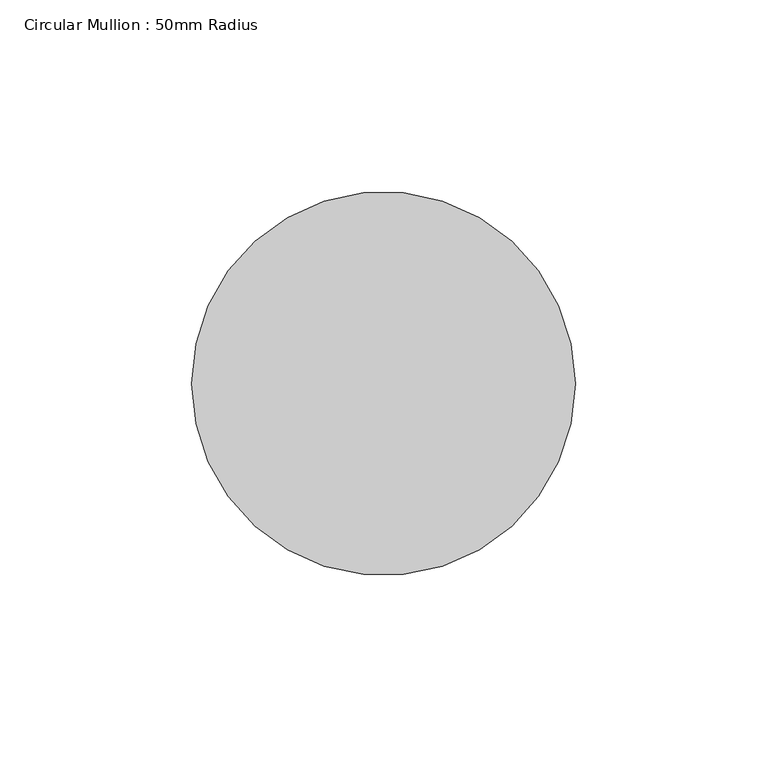
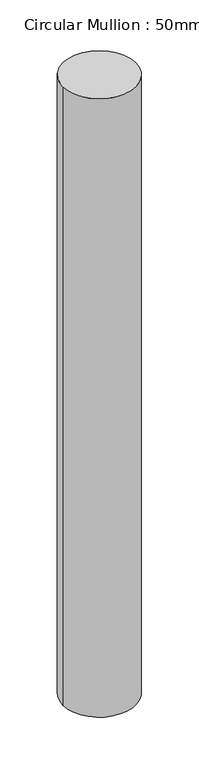
"""IFC4 building model written with IfcOpenShell, lengths in millimetres: member geometry, Circular Mullion : 50mm Radius."""

from ifc_helpers import new_model, si_unit, point, frame, origin, origin_2d, place, context, project, spatial, circle_curve, trimmed, segment, composite_curve, outline, extrude, source, transform, mapped, element, save


def circular_mullion_50mm_radius_ff912db3(model_context):
    return source(origin(), model_context, "Body", "SweptSolid", [
        extrude(outline(composite_curve([segment(trimmed(circle_curve(origin_2d(), 50.0), [point((50.0, 0.0))], [point((-50.0, 0.0))], False, "CARTESIAN"), True, "CONTINUOUS"), segment(trimmed(circle_curve(origin_2d(), 50.0), [point((-50.0, 0.0))], [point((50.0, 0.0))], False, "CARTESIAN"), True, "CONTINUOUS")], self_intersect=False)), frame((0.0, 0.0, -899.0118356), z_axis=(0.0, 0.0, 1.0), x_axis=(1.0, 0.0, 0.0)), (0.0, 0.0, 1.0), 899.0118356),
    ])


if __name__ == "__main__":
    model = new_model("IFC4")
    model_context = context("Model", 3, world=origin())
    ifc_project = project(units=[si_unit("LENGTHUNIT", "METRE", prefix="MILLI")], contexts=[model_context])
    site = spatial("IfcSite", under=ifc_project)
    building = spatial("IfcBuilding", under=site)
    placement = place(None, origin())
    circular_mullion_50mm_radius_shape = circular_mullion_50mm_radius_ff912db3(model_context)
    element("IfcMember", 1, ObjectType="Circular Mullion : 50mm Radius", at=placement, inside=building, context=model_context, shape_type="MappedRepresentation", body=[
        mapped(circular_mullion_50mm_radius_shape, transform((0.0, 0.0, 0.0), x_axis=(1.0, 0.0, 0.0), y_axis=(0.0, 1.0, 0.0), z_axis=(0.0, 0.0, 1.0))),
    ])
    save(model, "model.ifc")

# Revit data of these elements
# Type "Circular Mullion : 50mm Radius"
#   built-in parameter 1007350 = 0.164042 (stored number, unit not read)
# Element 1 (IfcMember, "Circular Mullion : 50mm Radius")
#   Materials on its faces: "Aluminium"
# Materials
#   "Aluminium": class "Metal", colour RGB 247 247 247, transparency 0, Description = "Aluminium 6061", Cost = 0
